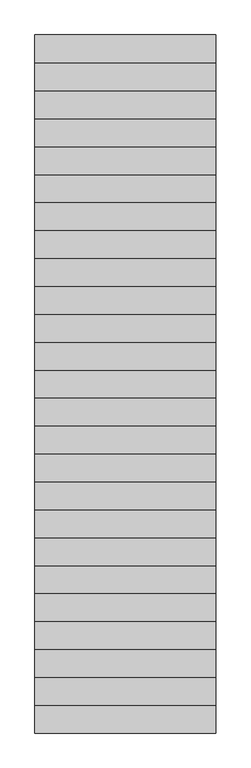
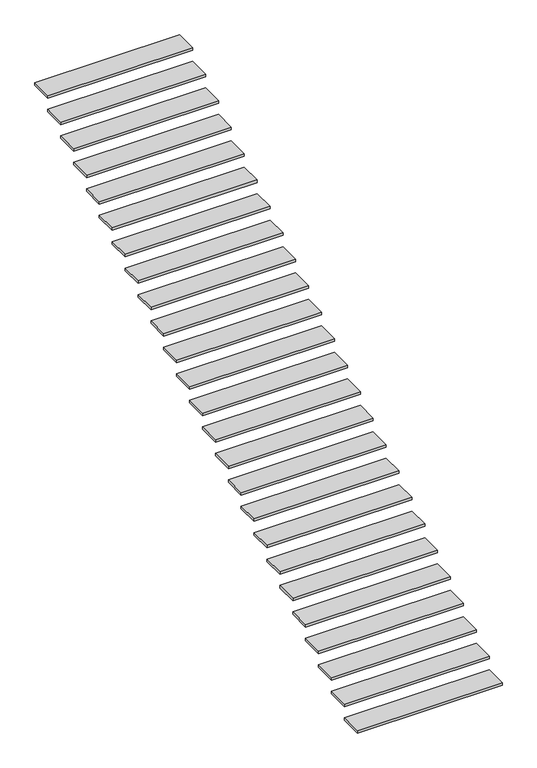
"""IFC4 building model written with IfcOpenShell, lengths in millimetres: stair flight geometry."""

import ifcopenshell
import ifcopenshell.guid

model = None  # the IFC model being written
_history = None  # IfcOwnerHistory: only IFC2X3 demands one
_inside = {}  # id of a spatial element -> (the spatial element, [elements in it])
_under = {}  # id of a project, library or spatial element -> (it, [spatial elements below it])
_declared = {}  # id of a project -> (the project, [libraries it declares])
_typed = {}  # id of a type object -> (the type object, [elements of that type])
_made_of = {}  # id of a material, layer set ... -> (it, [elements and type objects made of it])


def new_model(schema):
    """Start an empty IFC model of exactly this schema.

    Asked for "IFC4X3", IfcOpenShell would pick the latest addendum, in which some entities
    have other attributes; the version numbers below select the first issue.
    IFC2X3 requires an IfcOwnerHistory on every rooted entity: one is made here for all.
    """
    global model, _history
    if schema == "IFC4X3":
        model = ifcopenshell.file(schema_version=(4, 3, 0, 0))
    else:
        model = ifcopenshell.file(schema=schema)
    _inside.clear()
    _under.clear()
    _declared.clear()
    _typed.clear()
    _made_of.clear()
    _history = None
    if model.schema == "IFC2X3":
        org = make("IfcOrganization", Name="unknown")
        user = make(
            "IfcPersonAndOrganization",
            ThePerson=make("IfcPerson", FamilyName="unknown"),
            TheOrganization=org,
        )
        app = make(
            "IfcApplication",
            ApplicationDeveloper=org,
            Version="unknown",
            ApplicationFullName="unknown",
            ApplicationIdentifier="unknown",
        )
        _history = make(
            "IfcOwnerHistory",
            OwningUser=user,
            OwningApplication=app,
            ChangeAction="ADDED",
            CreationDate=0,
        )
    return model


def make(cls, **values):
    """One entity of the class cls with the attributes given. An attribute that is None is left unset."""
    return model.create_entity(
        cls, **{name: value for name, value in values.items() if value is not None}
    )


def rooted(cls, **values):
    """An entity with a GlobalId (a new one), such as an element, a storey or a relation."""
    return make(cls, GlobalId=ifcopenshell.guid.new(), OwnerHistory=_history, **values)


def si_unit(unit_type, name, prefix=None):
    """IfcSIUnit, for example si_unit("LENGTHUNIT", "METRE", prefix="MILLI")."""
    return make("IfcSIUnit", UnitType=unit_type, Prefix=prefix, Name=name)


def assignment(units):
    """IfcUnitAssignment: the units of a project."""
    return None if units is None else make("IfcUnitAssignment", Units=units)


def point(xyz):
    """IfcCartesianPoint."""
    return None if xyz is None else make("IfcCartesianPoint", Coordinates=xyz)


def direction(xyz):
    """IfcDirection."""
    return None if xyz is None else make("IfcDirection", DirectionRatios=xyz)


def frame(location, z_axis=None, x_axis=None):
    """IfcAxis2Placement3D, a coordinate frame: its origin and axes. An axis left out is left unset."""
    return make(
        "IfcAxis2Placement3D",
        Location=point(location),
        Axis=direction(z_axis),
        RefDirection=direction(x_axis),
    )


def origin():
    """The frame at (0, 0, 0) with its axes left unset."""
    return frame((0.0, 0.0, 0.0))


def place(relative_to, where):
    """IfcLocalPlacement: puts the frame where relative to a parent placement (None: the world)."""
    return make(
        "IfcLocalPlacement", PlacementRelTo=relative_to, RelativePlacement=where
    )


def context(
    kind, dimensions, precision=None, world=None, true_north=None, identifier=None
):
    """IfcGeometricRepresentationContext, for example the 3D "Model" context."""
    return make(
        "IfcGeometricRepresentationContext",
        ContextIdentifier=identifier,
        ContextType=kind,
        CoordinateSpaceDimension=dimensions,
        Precision=precision,
        WorldCoordinateSystem=world,
        TrueNorth=true_north,
    )


def project(units=None, contexts=None):
    """IfcProject with its units and contexts."""
    return rooted(
        "IfcProject",
        Name="project",
        RepresentationContexts=contexts,
        UnitsInContext=assignment(units),
    )


def spatial(cls, under=None, at=None, **own):
    """A site, building, storey or space (cls), placed at a placement, below another one or the project."""
    s = rooted(cls, ObjectPlacement=at, **own)
    if under is not None:
        _under.setdefault(under.id(), (under, []))[1].append(s)
    return s


def polyline(points):
    """IfcPolyline through the points."""
    return make("IfcPolyline", Points=[point(p) for p in points])


def outline(outer, holes=None, kind="AREA"):
    """IfcArbitraryClosedProfileDef: a profile drawn as a closed curve; with holes, ...WithVoids."""
    if holes is None:
        return make("IfcArbitraryClosedProfileDef", ProfileType=kind, OuterCurve=outer)
    return make(
        "IfcArbitraryProfileDefWithVoids",
        ProfileType=kind,
        OuterCurve=outer,
        InnerCurves=holes,
    )


def extrude(swept, where, along, depth):
    """IfcExtrudedAreaSolid: the profile swept, set in the frame where, extruded along a direction by depth."""
    return make(
        "IfcExtrudedAreaSolid",
        SweptArea=swept,
        Position=where,
        ExtrudedDirection=direction(along),
        Depth=depth,
    )


def shape(context_of_items, identifier, shape_type, items):
    """IfcShapeRepresentation: the items that make up one representation, for example the "Body"."""
    return make(
        "IfcShapeRepresentation",
        ContextOfItems=context_of_items,
        RepresentationIdentifier=identifier,
        RepresentationType=shape_type,
        Items=items,
    )


def source(mapping_origin, context_of_items, identifier, shape_type, items):
    """IfcRepresentationMap: a shape defined once, which mapped items show again and again."""
    return make(
        "IfcRepresentationMap",
        MappingOrigin=mapping_origin,
        MappedRepresentation=shape(context_of_items, identifier, shape_type, items),
    )


def transform(
    local_origin,
    x_axis=None,
    y_axis=None,
    z_axis=None,
    scale=None,
    scale2=None,
    scale3=None,
    uniform=True,
):
    """IfcCartesianTransformationOperator3D, or its non-uniform kind. x_axis, y_axis, z_axis: its Axis1, 2, 3."""
    if uniform:
        return make(
            "IfcCartesianTransformationOperator3D",
            Axis1=direction(x_axis),
            Axis2=direction(y_axis),
            LocalOrigin=point(local_origin),
            Scale=scale,
            Axis3=direction(z_axis),
        )
    return make(
        "IfcCartesianTransformationOperator3DnonUniform",
        Axis1=direction(x_axis),
        Axis2=direction(y_axis),
        LocalOrigin=point(local_origin),
        Scale=scale,
        Axis3=direction(z_axis),
        Scale2=scale2,
        Scale3=scale3,
    )


def mapped(mapping_source, mapping_target):
    """IfcMappedItem: shows the shape of a source again, moved by a transform."""
    return make(
        "IfcMappedItem", MappingSource=mapping_source, MappingTarget=mapping_target
    )


def made_of(thing, what):
    """Note that an element or type object is made of a material, layer set ...; save() writes the relation."""
    if what is not None:
        _made_of.setdefault(what.id(), (what, []))[1].append(thing)
    return thing


def element(
    cls,
    number,
    at=None,
    inside=None,
    cuts=None,
    type_object=None,
    material=None,
    context=None,
    identifier="Body",
    shape_type=None,
    held_by="IfcProductDefinitionShape",
    body=None,
    shapes=None,
    **own,
):
    """One element of the class cls, such as IfcWall. Its Tag is "e" and its number.

    at: its placement. inside: the storey or other place that contains it. cuts: it is an
    opening in that element (IfcRelVoidsElement). A single representation is given by context,
    identifier, shape_type and body (its items); several are given by shapes. held_by: the class
    of the entity that holds the representations. save() writes the other relations.
    """
    e = rooted(cls, Tag="e%d" % number, ObjectPlacement=at, **own)
    if body is not None:
        shapes = [shape(context, identifier, shape_type, body)]
    if shapes is not None:
        e.Representation = make(held_by, Representations=shapes)
    if inside is not None:
        _inside.setdefault(inside.id(), (inside, []))[1].append(e)
    if cuts is not None:
        rooted(
            "IfcRelVoidsElement", RelatingBuildingElement=cuts, RelatedOpeningElement=e
        )
    if type_object is not None:
        _typed.setdefault(type_object.id(), (type_object, []))[1].append(e)
    return made_of(e, material)


def aggregate(whole, parts):
    """IfcRelAggregates: a whole, such as a stair, and the parts it consists of."""
    return rooted("IfcRelAggregates", RelatingObject=whole, RelatedObjects=parts)


def save(model, path):
    """Write the relations noted so far, then the file.

    IfcRelAggregates (storeys below a building ...), IfcRelContainedInSpatialStructure (elements
    in a storey), IfcRelDefinesByType, IfcRelAssociatesMaterial and IfcRelDeclares: one each for
    every whole, place, type object, material and project.
    """
    for whole, parts in _under.values():
        aggregate(whole, parts)
    for where, things in _inside.values():
        rooted(
            "IfcRelContainedInSpatialStructure",
            RelatedElements=things,
            RelatingStructure=where,
        )
    for kind, things in _typed.values():
        rooted("IfcRelDefinesByType", RelatedObjects=things, RelatingType=kind)
    for what, things in _made_of.values():
        rooted("IfcRelAssociatesMaterial", RelatedObjects=things, RelatingMaterial=what)
    for by, libraries in _declared.values():
        rooted("IfcRelDeclares", RelatingContext=by, RelatedDefinitions=libraries)
    model.write(path)


def stair_flight_bdd207e3(model_context):
    return source(origin(), model_context, "Body", "SweptSolid", [
        extrude(outline(polyline([(17901.6097182, 11457.7630152), (19651.6097182, 11457.7630152), (19651.6097182, 11187.7630152), (17901.6097182, 11187.7630152), (17901.6097182, 11457.7630152)])), frame((0.0, 0.0, -158.0), z_axis=(0.0, 0.0, 1.0), x_axis=(1.0, 0.0, 0.0)), (0.0, 0.0, 1.0), 32.0),
        extrude(outline(polyline([(17901.6097182, 11727.7630152), (19651.6097182, 11727.7630152), (19651.6097182, 11457.7630152), (17901.6097182, 11457.7630152), (17901.6097182, 11727.7630152)])), frame((0.0, 0.0, 16.0), z_axis=(0.0, 0.0, 1.0), x_axis=(1.0, 0.0, 0.0)), (0.0, 0.0, 1.0), 32.0),
        extrude(outline(polyline([(17901.6097182, 11997.7630152), (19651.6097182, 11997.7630152), (19651.6097182, 11727.7630152), (17901.6097182, 11727.7630152), (17901.6097182, 11997.7630152)])), frame((0.0, 0.0, 190.0), z_axis=(0.0, 0.0, 1.0), x_axis=(1.0, 0.0, 0.0)), (0.0, 0.0, 1.0), 32.0),
        extrude(outline(polyline([(17901.6097182, 12267.7630152), (19651.6097182, 12267.7630152), (19651.6097182, 11997.7630152), (17901.6097182, 11997.7630152), (17901.6097182, 12267.7630152)])), frame((0.0, 0.0, 364.0), z_axis=(0.0, 0.0, 1.0), x_axis=(1.0, 0.0, 0.0)), (0.0, 0.0, 1.0), 32.0),
        extrude(outline(polyline([(17901.6097182, 12537.7630152), (19651.6097182, 12537.7630152), (19651.6097182, 12267.7630152), (17901.6097182, 12267.7630152), (17901.6097182, 12537.7630152)])), frame((0.0, 0.0, 538.0), z_axis=(0.0, 0.0, 1.0), x_axis=(1.0, 0.0, 0.0)), (0.0, 0.0, 1.0), 32.0),
        extrude(outline(polyline([(17901.6097182, 12807.7630152), (19651.6097182, 12807.7630152), (19651.6097182, 12537.7630152), (17901.6097182, 12537.7630152), (17901.6097182, 12807.7630152)])), frame((0.0, 0.0, 712.0), z_axis=(0.0, 0.0, 1.0), x_axis=(1.0, 0.0, 0.0)), (0.0, 0.0, 1.0), 32.0),
        extrude(outline(polyline([(17901.6097182, 13077.7630152), (19651.6097182, 13077.7630152), (19651.6097182, 12807.7630152), (17901.6097182, 12807.7630152), (17901.6097182, 13077.7630152)])), frame((0.0, 0.0, 886.0), z_axis=(0.0, 0.0, 1.0), x_axis=(1.0, 0.0, 0.0)), (0.0, 0.0, 1.0), 32.0),
        extrude(outline(polyline([(17901.6097182, 13347.7630152), (19651.6097182, 13347.7630152), (19651.6097182, 13077.7630152), (17901.6097182, 13077.7630152), (17901.6097182, 13347.7630152)])), frame((0.0, 0.0, 1060.0), z_axis=(0.0, 0.0, 1.0), x_axis=(1.0, 0.0, 0.0)), (0.0, 0.0, 1.0), 32.0),
        extrude(outline(polyline([(17901.6097182, 13617.7630152), (19651.6097182, 13617.7630152), (19651.6097182, 13347.7630152), (17901.6097182, 13347.7630152), (17901.6097182, 13617.7630152)])), frame((0.0, 0.0, 1234.0), z_axis=(0.0, 0.0, 1.0), x_axis=(1.0, 0.0, 0.0)), (0.0, 0.0, 1.0), 32.0),
        extrude(outline(polyline([(17901.6097182, 13887.7630152), (19651.6097182, 13887.7630152), (19651.6097182, 13617.7630152), (17901.6097182, 13617.7630152), (17901.6097182, 13887.7630152)])), frame((0.0, 0.0, 1408.0), z_axis=(0.0, 0.0, 1.0), x_axis=(1.0, 0.0, 0.0)), (0.0, 0.0, 1.0), 32.0),
        extrude(outline(polyline([(17901.6097182, 14157.7630152), (19651.6097182, 14157.7630152), (19651.6097182, 13887.7630152), (17901.6097182, 13887.7630152), (17901.6097182, 14157.7630152)])), frame((0.0, 0.0, 1582.0), z_axis=(0.0, 0.0, 1.0), x_axis=(1.0, 0.0, 0.0)), (0.0, 0.0, 1.0), 32.0),
        extrude(outline(polyline([(17901.6097182, 14427.7630152), (19651.6097182, 14427.7630152), (19651.6097182, 14157.7630152), (17901.6097182, 14157.7630152), (17901.6097182, 14427.7630152)])), frame((0.0, 0.0, 1756.0), z_axis=(0.0, 0.0, 1.0), x_axis=(1.0, 0.0, 0.0)), (0.0, 0.0, 1.0), 32.0),
        extrude(outline(polyline([(17901.6097182, 14697.7630152), (19651.6097182, 14697.7630152), (19651.6097182, 14427.7630152), (17901.6097182, 14427.7630152), (17901.6097182, 14697.7630152)])), frame((0.0, 0.0, 1930.0), z_axis=(0.0, 0.0, 1.0), x_axis=(1.0, 0.0, 0.0)), (0.0, 0.0, 1.0), 32.0),
        extrude(outline(polyline([(17901.6097182, 14967.7630152), (19651.6097182, 14967.7630152), (19651.6097182, 14697.7630152), (17901.6097182, 14697.7630152), (17901.6097182, 14967.7630152)])), frame((0.0, 0.0, 2104.0), z_axis=(0.0, 0.0, 1.0), x_axis=(1.0, 0.0, 0.0)), (0.0, 0.0, 1.0), 32.0),
        extrude(outline(polyline([(17901.6097182, 15237.7630152), (19651.6097182, 15237.7630152), (19651.6097182, 14967.7630152), (17901.6097182, 14967.7630152), (17901.6097182, 15237.7630152)])), frame((0.0, 0.0, 2278.0), z_axis=(0.0, 0.0, 1.0), x_axis=(1.0, 0.0, 0.0)), (0.0, 0.0, 1.0), 32.0),
        extrude(outline(polyline([(17901.6097182, 15507.7630152), (19651.6097182, 15507.7630152), (19651.6097182, 15237.7630152), (17901.6097182, 15237.7630152), (17901.6097182, 15507.7630152)])), frame((0.0, 0.0, 2452.0), z_axis=(0.0, 0.0, 1.0), x_axis=(1.0, 0.0, 0.0)), (0.0, 0.0, 1.0), 32.0),
        extrude(outline(polyline([(17901.6097182, 15777.7630152), (19651.6097182, 15777.7630152), (19651.6097182, 15507.7630152), (17901.6097182, 15507.7630152), (17901.6097182, 15777.7630152)])), frame((0.0, 0.0, 2626.0), z_axis=(0.0, 0.0, 1.0), x_axis=(1.0, 0.0, 0.0)), (0.0, 0.0, 1.0), 32.0),
        extrude(outline(polyline([(17901.6097182, 16047.7630152), (19651.6097182, 16047.7630152), (19651.6097182, 15777.7630152), (17901.6097182, 15777.7630152), (17901.6097182, 16047.7630152)])), frame((0.0, 0.0, 2800.0), z_axis=(0.0, 0.0, 1.0), x_axis=(1.0, 0.0, 0.0)), (0.0, 0.0, 1.0), 32.0),
        extrude(outline(polyline([(17901.6097182, 16317.7630152), (19651.6097182, 16317.7630152), (19651.6097182, 16047.7630152), (17901.6097182, 16047.7630152), (17901.6097182, 16317.7630152)])), frame((0.0, 0.0, 2974.0), z_axis=(0.0, 0.0, 1.0), x_axis=(1.0, 0.0, 0.0)), (0.0, 0.0, 1.0), 32.0),
        extrude(outline(polyline([(17901.6097182, 16587.7630152), (19651.6097182, 16587.7630152), (19651.6097182, 16317.7630152), (17901.6097182, 16317.7630152), (17901.6097182, 16587.7630152)])), frame((0.0, 0.0, 3148.0), z_axis=(0.0, 0.0, 1.0), x_axis=(1.0, 0.0, 0.0)), (0.0, 0.0, 1.0), 32.0),
        extrude(outline(polyline([(17901.6097182, 16857.7630152), (19651.6097182, 16857.7630152), (19651.6097182, 16587.7630152), (17901.6097182, 16587.7630152), (17901.6097182, 16857.7630152)])), frame((0.0, 0.0, 3322.0), z_axis=(0.0, 0.0, 1.0), x_axis=(1.0, 0.0, 0.0)), (0.0, 0.0, 1.0), 32.0),
        extrude(outline(polyline([(17901.6097182, 17127.7630152), (19651.6097182, 17127.7630152), (19651.6097182, 16857.7630152), (17901.6097182, 16857.7630152), (17901.6097182, 17127.7630152)])), frame((0.0, 0.0, 3496.0), z_axis=(0.0, 0.0, 1.0), x_axis=(1.0, 0.0, 0.0)), (0.0, 0.0, 1.0), 32.0),
        extrude(outline(polyline([(17901.6097182, 17397.7630152), (19651.6097182, 17397.7630152), (19651.6097182, 17127.7630152), (17901.6097182, 17127.7630152), (17901.6097182, 17397.7630152)])), frame((0.0, 0.0, 3670.0), z_axis=(0.0, 0.0, 1.0), x_axis=(1.0, 0.0, 0.0)), (0.0, 0.0, 1.0), 32.0),
        extrude(outline(polyline([(17901.6097182, 17667.7630152), (19651.6097182, 17667.7630152), (19651.6097182, 17397.7630152), (17901.6097182, 17397.7630152), (17901.6097182, 17667.7630152)])), frame((0.0, 0.0, 3844.0), z_axis=(0.0, 0.0, 1.0), x_axis=(1.0, 0.0, 0.0)), (0.0, 0.0, 1.0), 32.0),
        extrude(outline(polyline([(17901.6097182, 17937.7630152), (19651.6097182, 17937.7630152), (19651.6097182, 17667.7630152), (17901.6097182, 17667.7630152), (17901.6097182, 17937.7630152)])), frame((0.0, 0.0, 4018.0), z_axis=(0.0, 0.0, 1.0), x_axis=(1.0, 0.0, 0.0)), (0.0, 0.0, 1.0), 32.0),
    ])


if __name__ == "__main__":
    model = new_model("IFC4")
    model_context = context("Model", 3, world=origin())
    ifc_project = project(units=[si_unit("LENGTHUNIT", "METRE", prefix="MILLI")], contexts=[model_context])
    site = spatial("IfcSite", under=ifc_project)
    building = spatial("IfcBuilding", under=site)
    placement = place(None, origin())
    stair_flight_shape = stair_flight_bdd207e3(model_context)
    element("IfcStairFlight", 1, at=placement, inside=building, context=model_context, shape_type="MappedRepresentation", body=[
        mapped(stair_flight_shape, transform((0.0, 0.0, 0.0), x_axis=(1.0, 0.0, 0.0), y_axis=(0.0, 1.0, 0.0), z_axis=(0.0, 0.0, 1.0))),
    ])
    save(model, "model.ifc")

# Revit data of these elements
# Element 1 (IfcStairFlight)
#   Materials on its faces: "철강"
# Materials
#   "철강": class "Generic", colour RGB 143 142 141, transparency 0, Description = "철골+가공조립+세우기", Cost = 0
